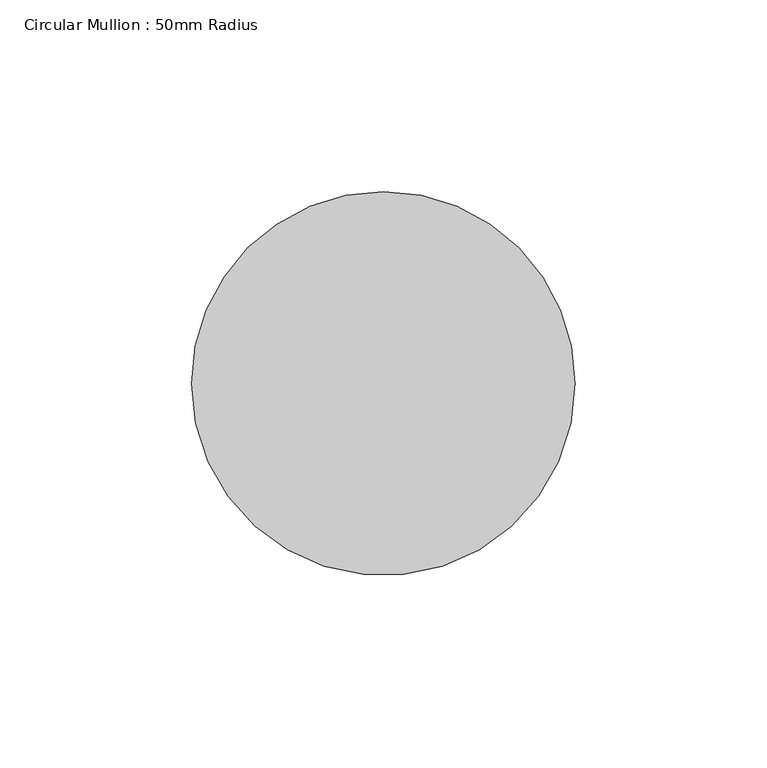
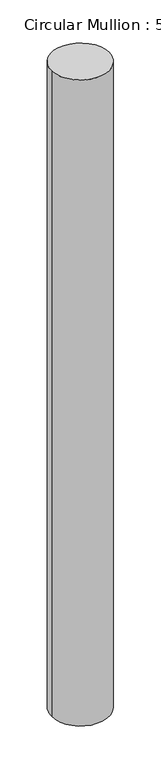
"""IFC4 building model written with IfcOpenShell, lengths in millimetres: member geometry, Circular Mullion : 50mm Radius."""

from ifc_helpers import new_model, si_unit, frame, origin, place, context, project, spatial, ellipse_curve, source, transform, mapped, element, save
from ifc_brep_helpers import plane_surface, cylinder_surface, advanced_brep


def circular_mullion_50mm_radius_61a615d9(model_context):
    return source(origin(), model_context, "Body", "AdvancedBrep", [
        advanced_brep(
        [(-100.0, 0.0, 0.9395667), (0.0, 0.0, 0.0), (0.0, 0.0, -1183.1509022), (-100.0, 0.0, -1184.1477213)],
        [
            (0, 1, ellipse_curve(frame((-50.0, 0.0, 0.4697833), z_axis=(-0.009393522396021712, -0.019187285559301815, -0.9997717788624869), x_axis=(-0.43960355739669665, -0.8979378164071444, 0.02136329071417454)), 50.0114137, 50.0)),
            (1, 2),
            (2, 3, ellipse_curve(frame((-50.0, 0.0, -1183.6493118), z_axis=(-0.009965630422987596, -0.02035587808736212, 0.9997431292274856), x_axis=(0.43959096004025844, 0.8979120849439823, 0.02266441180429866)), 50.0128468, 50.0)),
            (3, 0),
            (1, 0, ellipse_curve(frame((-50.0, 0.0, 0.4697833), z_axis=(-0.009393522396021712, -0.019187285559301815, -0.9997717788624869), x_axis=(-0.43960355739669665, -0.8979378164071444, 0.02136329071417454)), 50.0114137, 50.0)),
            (3, 2, ellipse_curve(frame((-50.0, 0.0, -1183.6493118), z_axis=(-0.009965630422987596, -0.02035587808736212, 0.9997431292274856), x_axis=(0.43959096004025844, 0.8979120849439823, 0.02266441180429866)), 50.0128468, 50.0)),
        ],
        [
            cylinder_surface(frame((-50.0, 0.0, 0.0), z_axis=(0.0, 0.0, 1.0), x_axis=(1.0, 0.0, 0.0)), 50.0),
            plane_surface(frame((-273.7539229, 134.0217509, 0.0), z_axis=(0.009393522396021712, 0.019187285559301815, 0.9997717788624869), x_axis=(0.4396035573966976, 0.897937816407144, -0.021363290714184306))),
            plane_surface(frame((-273.7539229, 134.0217509, -1183.1509022), z_axis=(0.009965630422987596, 0.02035587808736212, -0.9997431292274856), x_axis=(0.43959096004025844, 0.8979120849439821, 0.022664411804305118))),
        ],
        [
            (0, [[1, 2, 3, 4]]),
            (0, [[5, -4, 6, -2]]),
            (1, [[-1, -5]]),
            (2, [[-6, -3]]),
        ],
    ),
    ])


if __name__ == "__main__":
    model = new_model("IFC4")
    model_context = context("Model", 3, world=origin())
    ifc_project = project(units=[si_unit("LENGTHUNIT", "METRE", prefix="MILLI")], contexts=[model_context])
    site = spatial("IfcSite", under=ifc_project)
    building = spatial("IfcBuilding", under=site)
    placement = place(None, origin())
    circular_mullion_50mm_radius_shape = circular_mullion_50mm_radius_61a615d9(model_context)
    element("IfcMember", 1, ObjectType="Circular Mullion : 50mm Radius", at=placement, inside=building, context=model_context, shape_type="MappedRepresentation", body=[
        mapped(circular_mullion_50mm_radius_shape, transform((0.0, 0.0, 0.0), x_axis=(1.0, 0.0, 0.0), y_axis=(0.0, 1.0, 0.0), z_axis=(0.0, 0.0, 1.0))),
    ])
    save(model, "model.ifc")

# Revit data of these elements
# Type "Circular Mullion : 50mm Radius"
#   built-in parameter 1007350 = 0.164042 (stored number, unit not read)
# Element 1 (IfcMember, "Circular Mullion : 50mm Radius")
#   Materials on its faces: "Aluminium"
# Materials
#   "Aluminium": class "Metal", colour RGB 247 247 247, transparency 0, Description = "Aluminium 6061", Cost = 0
